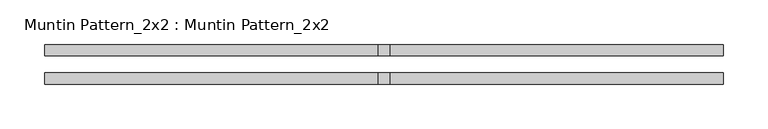
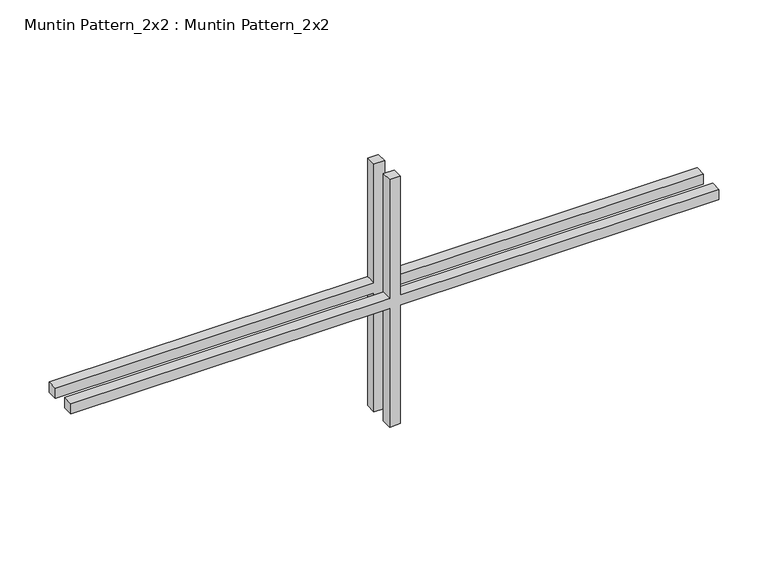
"""IFC4 building model written with IfcOpenShell, lengths in millimetres: proxy geometry, Muntin Pattern_2x2 : Muntin Pattern_2x2."""

import ifcopenshell
import ifcopenshell.guid

model = None  # the IFC model being written
_history = None  # IfcOwnerHistory: only IFC2X3 demands one
_inside = {}  # id of a spatial element -> (the spatial element, [elements in it])
_under = {}  # id of a project, library or spatial element -> (it, [spatial elements below it])
_declared = {}  # id of a project -> (the project, [libraries it declares])
_typed = {}  # id of a type object -> (the type object, [elements of that type])
_made_of = {}  # id of a material, layer set ... -> (it, [elements and type objects made of it])


def new_model(schema):
    """Start an empty IFC model of exactly this schema.

    Asked for "IFC4X3", IfcOpenShell would pick the latest addendum, in which some entities
    have other attributes; the version numbers below select the first issue.
    IFC2X3 requires an IfcOwnerHistory on every rooted entity: one is made here for all.
    """
    global model, _history
    if schema == "IFC4X3":
        model = ifcopenshell.file(schema_version=(4, 3, 0, 0))
    else:
        model = ifcopenshell.file(schema=schema)
    _inside.clear()
    _under.clear()
    _declared.clear()
    _typed.clear()
    _made_of.clear()
    _history = None
    if model.schema == "IFC2X3":
        org = make("IfcOrganization", Name="unknown")
        user = make(
            "IfcPersonAndOrganization",
            ThePerson=make("IfcPerson", FamilyName="unknown"),
            TheOrganization=org,
        )
        app = make(
            "IfcApplication",
            ApplicationDeveloper=org,
            Version="unknown",
            ApplicationFullName="unknown",
            ApplicationIdentifier="unknown",
        )
        _history = make(
            "IfcOwnerHistory",
            OwningUser=user,
            OwningApplication=app,
            ChangeAction="ADDED",
            CreationDate=0,
        )
    return model


def make(cls, **values):
    """One entity of the class cls with the attributes given. An attribute that is None is left unset."""
    return model.create_entity(
        cls, **{name: value for name, value in values.items() if value is not None}
    )


def rooted(cls, **values):
    """An entity with a GlobalId (a new one), such as an element, a storey or a relation."""
    return make(cls, GlobalId=ifcopenshell.guid.new(), OwnerHistory=_history, **values)


def si_unit(unit_type, name, prefix=None):
    """IfcSIUnit, for example si_unit("LENGTHUNIT", "METRE", prefix="MILLI")."""
    return make("IfcSIUnit", UnitType=unit_type, Prefix=prefix, Name=name)


def assignment(units):
    """IfcUnitAssignment: the units of a project."""
    return None if units is None else make("IfcUnitAssignment", Units=units)


def point(xyz):
    """IfcCartesianPoint."""
    return None if xyz is None else make("IfcCartesianPoint", Coordinates=xyz)


def direction(xyz):
    """IfcDirection."""
    return None if xyz is None else make("IfcDirection", DirectionRatios=xyz)


def frame(location, z_axis=None, x_axis=None):
    """IfcAxis2Placement3D, a coordinate frame: its origin and axes. An axis left out is left unset."""
    return make(
        "IfcAxis2Placement3D",
        Location=point(location),
        Axis=direction(z_axis),
        RefDirection=direction(x_axis),
    )


def origin():
    """The frame at (0, 0, 0) with its axes left unset."""
    return frame((0.0, 0.0, 0.0))


def place(relative_to, where):
    """IfcLocalPlacement: puts the frame where relative to a parent placement (None: the world)."""
    return make(
        "IfcLocalPlacement", PlacementRelTo=relative_to, RelativePlacement=where
    )


def context(
    kind, dimensions, precision=None, world=None, true_north=None, identifier=None
):
    """IfcGeometricRepresentationContext, for example the 3D "Model" context."""
    return make(
        "IfcGeometricRepresentationContext",
        ContextIdentifier=identifier,
        ContextType=kind,
        CoordinateSpaceDimension=dimensions,
        Precision=precision,
        WorldCoordinateSystem=world,
        TrueNorth=true_north,
    )


def project(units=None, contexts=None):
    """IfcProject with its units and contexts."""
    return rooted(
        "IfcProject",
        Name="project",
        RepresentationContexts=contexts,
        UnitsInContext=assignment(units),
    )


def spatial(cls, under=None, at=None, **own):
    """A site, building, storey or space (cls), placed at a placement, below another one or the project."""
    s = rooted(cls, ObjectPlacement=at, **own)
    if under is not None:
        _under.setdefault(under.id(), (under, []))[1].append(s)
    return s


def polyline(points):
    """IfcPolyline through the points."""
    return make("IfcPolyline", Points=[point(p) for p in points])


def outline(outer, holes=None, kind="AREA"):
    """IfcArbitraryClosedProfileDef: a profile drawn as a closed curve; with holes, ...WithVoids."""
    if holes is None:
        return make("IfcArbitraryClosedProfileDef", ProfileType=kind, OuterCurve=outer)
    return make(
        "IfcArbitraryProfileDefWithVoids",
        ProfileType=kind,
        OuterCurve=outer,
        InnerCurves=holes,
    )


def extrude(swept, where, along, depth):
    """IfcExtrudedAreaSolid: the profile swept, set in the frame where, extruded along a direction by depth."""
    return make(
        "IfcExtrudedAreaSolid",
        SweptArea=swept,
        Position=where,
        ExtrudedDirection=direction(along),
        Depth=depth,
    )


def shape(context_of_items, identifier, shape_type, items):
    """IfcShapeRepresentation: the items that make up one representation, for example the "Body"."""
    return make(
        "IfcShapeRepresentation",
        ContextOfItems=context_of_items,
        RepresentationIdentifier=identifier,
        RepresentationType=shape_type,
        Items=items,
    )


def source(mapping_origin, context_of_items, identifier, shape_type, items):
    """IfcRepresentationMap: a shape defined once, which mapped items show again and again."""
    return make(
        "IfcRepresentationMap",
        MappingOrigin=mapping_origin,
        MappedRepresentation=shape(context_of_items, identifier, shape_type, items),
    )


def transform(
    local_origin,
    x_axis=None,
    y_axis=None,
    z_axis=None,
    scale=None,
    scale2=None,
    scale3=None,
    uniform=True,
):
    """IfcCartesianTransformationOperator3D, or its non-uniform kind. x_axis, y_axis, z_axis: its Axis1, 2, 3."""
    if uniform:
        return make(
            "IfcCartesianTransformationOperator3D",
            Axis1=direction(x_axis),
            Axis2=direction(y_axis),
            LocalOrigin=point(local_origin),
            Scale=scale,
            Axis3=direction(z_axis),
        )
    return make(
        "IfcCartesianTransformationOperator3DnonUniform",
        Axis1=direction(x_axis),
        Axis2=direction(y_axis),
        LocalOrigin=point(local_origin),
        Scale=scale,
        Axis3=direction(z_axis),
        Scale2=scale2,
        Scale3=scale3,
    )


def mapped(mapping_source, mapping_target):
    """IfcMappedItem: shows the shape of a source again, moved by a transform."""
    return make(
        "IfcMappedItem", MappingSource=mapping_source, MappingTarget=mapping_target
    )


def made_of(thing, what):
    """Note that an element or type object is made of a material, layer set ...; save() writes the relation."""
    if what is not None:
        _made_of.setdefault(what.id(), (what, []))[1].append(thing)
    return thing


def element(
    cls,
    number,
    at=None,
    inside=None,
    cuts=None,
    type_object=None,
    material=None,
    context=None,
    identifier="Body",
    shape_type=None,
    held_by="IfcProductDefinitionShape",
    body=None,
    shapes=None,
    **own,
):
    """One element of the class cls, such as IfcWall. Its Tag is "e" and its number.

    at: its placement. inside: the storey or other place that contains it. cuts: it is an
    opening in that element (IfcRelVoidsElement). A single representation is given by context,
    identifier, shape_type and body (its items); several are given by shapes. held_by: the class
    of the entity that holds the representations. save() writes the other relations.
    """
    e = rooted(cls, Tag="e%d" % number, ObjectPlacement=at, **own)
    if body is not None:
        shapes = [shape(context, identifier, shape_type, body)]
    if shapes is not None:
        e.Representation = make(held_by, Representations=shapes)
    if inside is not None:
        _inside.setdefault(inside.id(), (inside, []))[1].append(e)
    if cuts is not None:
        rooted(
            "IfcRelVoidsElement", RelatingBuildingElement=cuts, RelatedOpeningElement=e
        )
    if type_object is not None:
        _typed.setdefault(type_object.id(), (type_object, []))[1].append(e)
    return made_of(e, material)


def aggregate(whole, parts):
    """IfcRelAggregates: a whole, such as a stair, and the parts it consists of."""
    return rooted("IfcRelAggregates", RelatingObject=whole, RelatedObjects=parts)


def save(model, path):
    """Write the relations noted so far, then the file.

    IfcRelAggregates (storeys below a building ...), IfcRelContainedInSpatialStructure (elements
    in a storey), IfcRelDefinesByType, IfcRelAssociatesMaterial and IfcRelDeclares: one each for
    every whole, place, type object, material and project.
    """
    for whole, parts in _under.values():
        aggregate(whole, parts)
    for where, things in _inside.values():
        rooted(
            "IfcRelContainedInSpatialStructure",
            RelatedElements=things,
            RelatingStructure=where,
        )
    for kind, things in _typed.values():
        rooted("IfcRelDefinesByType", RelatedObjects=things, RelatingType=kind)
    for what, things in _made_of.values():
        rooted("IfcRelAssociatesMaterial", RelatedObjects=things, RelatingMaterial=what)
    for by, libraries in _declared.values():
        rooted("IfcRelDeclares", RelatingContext=by, RelatedDefinitions=libraries)
    model.write(path)


def muntin_pattern_2x2_muntin_pattern_2x2_101ea2c0(model_context):
    return source(origin(), model_context, "Body", "SweptSolid", [
        extrude(outline(polyline([(160.3375, -6.35), (160.3375, -381.0), (147.6375, -381.0), (147.6375, -6.35), (0.0, -6.35), (0.0, 6.35), (147.6375, 6.35), (147.6375, 381.0), (160.3375, 381.0), (160.3375, 6.35), (307.975, 6.35), (307.975, -6.35), (160.3375, -6.35)])), frame((0.0, 9.525, 0.0), z_axis=(0.0, 1.0, 0.0), x_axis=(0.0, 0.0, 1.0)), (0.0, 0.0, 1.0), 12.7),
        extrude(outline(polyline([(160.3375, -6.35), (160.3375, -381.0), (147.6375, -381.0), (147.6375, -6.35), (0.0, -6.35), (0.0, 6.35), (147.6375, 6.35), (147.6375, 381.0), (160.3375, 381.0), (160.3375, 6.35), (307.975, 6.35), (307.975, -6.35), (160.3375, -6.35)])), frame((0.0, -22.225, 0.0), z_axis=(0.0, 1.0, 0.0), x_axis=(0.0, 0.0, 1.0)), (0.0, 0.0, 1.0), 12.7),
    ])


if __name__ == "__main__":
    model = new_model("IFC4")
    model_context = context("Model", 3, world=origin())
    ifc_project = project(units=[si_unit("LENGTHUNIT", "METRE", prefix="MILLI")], contexts=[model_context])
    site = spatial("IfcSite", under=ifc_project)
    building = spatial("IfcBuilding", under=site)
    placement = place(None, origin())
    muntin_pattern_2x2_muntin_pattern_2x2_shape = muntin_pattern_2x2_muntin_pattern_2x2_101ea2c0(model_context)
    element("IfcBuildingElementProxy", 1, Name="Muntin Pattern_2x2 : Muntin Pattern_2x2", ObjectType="Muntin Pattern_2x2 : Muntin Pattern_2x2", at=placement, inside=building, context=model_context, shape_type="MappedRepresentation", body=[
        mapped(muntin_pattern_2x2_muntin_pattern_2x2_shape, transform((0.0, 0.0, 0.0), x_axis=(1.0, 0.0, 0.0), y_axis=(0.0, 1.0, 0.0), z_axis=(0.0, 0.0, 1.0))),
    ])
    save(model, "model.ifc")

# Revit data of these elements
# Type "Muntin Pattern_2x2 : Muntin Pattern_2x2"
#   Width [instance default] = 4' - 0"
#   Thickness = 0' - 0 1/2"
#   Height [instance default] = 4' - 0"
#   Distance = 0' - 0 3/4"
#   Interior Material [instance default] = none
#   Exterior Material [instance default] = none
#   Default Elevation = 0
# Element 1 (IfcBuildingElementProxy, "Muntin Pattern_2x2 : Muntin Pattern_2x2")
#   Width = 2' - 6"
#   Height = 1' - 0 1/8"
#   Interior Material = Wood - Stained
#   Exterior Material = Clad - White
#   Materials on its faces: "Clad - White", "Wood - Stained"
# Materials
#   "Clad - White": class "Wood", colour RGB 242 242 238, transparency 0, Cost = 0
#   "Wood - Stained": class "Wood", colour RGB 224 178 126, transparency 0, Cost = 0
